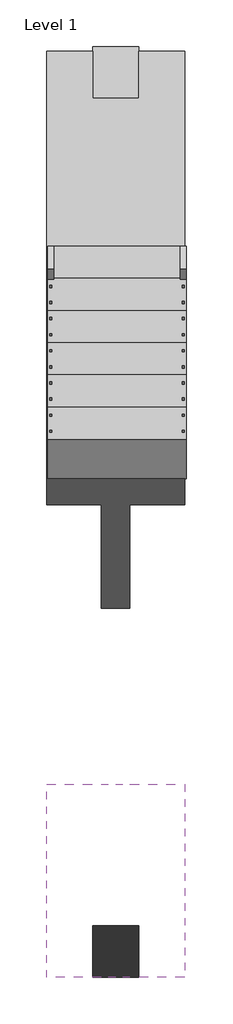
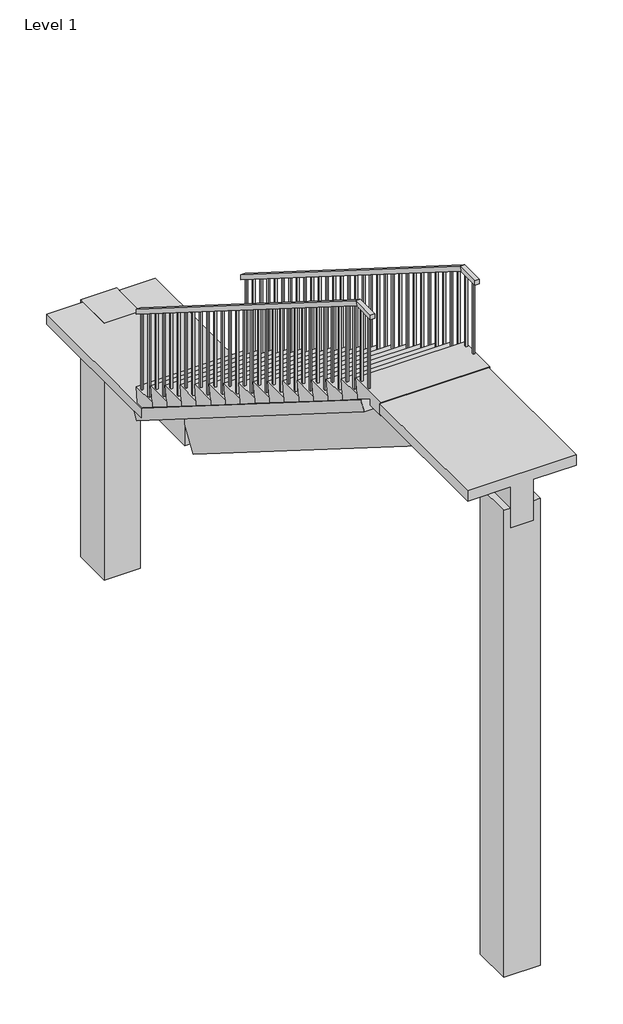
# One storey: 3 beams, 2 columns, 2 railings, 1 stair flight.
"""IFC4 building model written with IfcOpenShell, lengths in millimetres."""

from ifc_helpers import new_model, si_unit, frame, origin, place, context, project, spatial, polyline, outline, extrude, faceted_brep, element, save

model = new_model("IFC4")

# Units and contexts
model_context = context("Model", 3, world=origin())
ifc_project = project(units=[si_unit("LENGTHUNIT", "METRE", prefix="MILLI")], contexts=[model_context])

# Site, building, storey
site = spatial("IfcSite", under=ifc_project)
building = spatial("IfcBuilding", under=site)
storey = spatial("IfcBuildingStorey", under=building, Name="Level 1", Elevation=0.0)

# Beams
placement = place(None, origin())
element("IfcBeam", 1, ObjectType="Concrete-TRectangular Beam : b= 1200 x bw= 250 x tw= 120 x h=600 2", at=placement, inside=storey, context=model_context, shape_type="Brep", body=[
    faceted_brep([(2146.615308, 1121.0694774, 2541.613649), (2621.615308, 1121.0694774, 2541.613649), (2621.615308, 865.187293, 2135.5049102), (2871.615308, 865.187293, 2135.5049102), (2871.615308, 1121.0694774, 2541.613649), (3346.615308, 1121.0694774, 2541.613649), (3346.615308, 1185.0400235, 2643.1408337), (2146.615308, 1185.0400235, 2643.1408337), (3346.615308, 5379.9494631, 0.0), (2146.615308, 5379.9494631, 0.0), (3346.615308, 5468.6287248, -197.7092229), (3346.615308, 5517.5919797, -120.0), (3346.615308, 5373.0854091, -120.0), (3346.615308, 5373.0854091, 0.0), (2871.615308, 5373.0854091, -137.5090106), (2871.615308, 5468.6287248, -197.7092229), (2871.615308, 5212.7465404, -603.8179618), (2871.615308, 5373.0854091, -349.3453188), (2621.615308, 5212.7465404, -603.8179618), (2621.615308, 5373.0854091, -137.5090106), (2621.615308, 5373.0854091, -349.3453188), (2146.615308, 5468.6287248, -197.7092229), (2621.615308, 5468.6287248, -197.7092229), (2146.615308, 5373.0854091, 0.0), (2146.615308, 5373.0854091, -120.0), (2146.615308, 5517.5919797, -120.0), (2621.615308, 5517.5919797, -120.0), (2871.615308, 5373.0854091, -120.0), (2871.615308, 5517.5919797, -120.0), (2621.615308, 5373.0854091, -120.0)], [[[0, 1, 2, 3, 4, 5, 6, 7]], [[7, 6, 8, 9]], [[6, 5, 10, 11, 12, 13, 8]], [[5, 4, 14, 15, 10]], [[4, 3, 16, 17, 14]], [[3, 2, 18, 16]], [[2, 1, 19, 20, 18]], [[1, 0, 21, 22, 19]], [[0, 7, 9, 23, 24, 25, 21]], [[22, 21, 25, 26]], [[13, 23, 9, 8]], [[27, 12, 11, 28]], [[14, 27, 28, 15]], [[29, 19, 22, 26]], [[24, 29, 26, 25]], [[23, 13, 12, 27, 14, 17, 20, 19, 29, 24]], [[16, 18, 20, 17]], [[10, 15, 28, 11]]]),
])
element("IfcBeam", 2, ObjectType="Concrete-TRectangular Beam : b= 1200 x bw= 250 x tw= 120 x h=600 2", at=placement, inside=storey, context=model_context, shape_type="Brep", body=[
    faceted_brep([(2146.615308, 7193.0854091, 0.0), (2146.615308, 5379.9494631, 0.0), (2146.615308, 5373.0854091, 0.0), (3346.615308, 5373.0854091, 0.0), (3346.615308, 5379.9494631, 0.0), (3346.615308, 7193.0854091, 0.0), (2946.615308, 7193.0854091, 0.0), (2946.615308, 6785.5854091, 0.0), (2546.615308, 6785.5854091, 0.0), (2546.615308, 7193.0854091, 0.0), (3346.615308, 5373.0854091, -120.0), (3346.615308, 5517.5919797, -120.0), (3346.615308, 7193.0854091, -120.0), (2871.615308, 5373.0854091, -120.0), (2871.615308, 5517.5919797, -120.0), (2871.615308, 6785.5854091, -120.0), (2946.615308, 6785.5854091, -120.0), (2946.615308, 7193.0854091, -120.0), (2871.615308, 5373.0854091, -137.5090106), (2871.615308, 5373.0854091, -349.3453188), (2871.615308, 5373.0854091, -600.0), (2871.615308, 6785.5854091, -600.0), (2621.615308, 5373.0854091, -600.0), (2621.615308, 6785.5854091, -600.0), (2621.615308, 5373.0854091, -349.3453188), (2621.615308, 5373.0854091, -137.5090106), (2621.615308, 5373.0854091, -120.0), (2621.615308, 5517.5919797, -120.0), (2621.615308, 6785.5854091, -120.0), (2146.615308, 5373.0854091, -120.0), (2146.615308, 5517.5919797, -120.0), (2146.615308, 7193.0854091, -120.0), (2546.615308, 7193.0854091, -120.0), (2546.615308, 6785.5854091, -120.0)], [[[0, 1, 2, 3, 4, 5, 6, 7, 8, 9]], [[5, 4, 3, 10, 11, 12]], [[12, 11, 10, 13, 14, 15, 16, 17]], [[13, 18, 19, 20, 21, 15, 14]], [[20, 22, 23, 21]], [[22, 24, 25, 26, 27, 28, 23]], [[29, 30, 31, 32, 33, 28, 27, 26]], [[2, 1, 0, 31, 30, 29]], [[8, 33, 32, 9]], [[33, 8, 7, 16, 15, 21, 23, 28]], [[16, 7, 6, 17]], [[5, 12, 17, 6]], [[31, 0, 9, 32]], [[2, 29, 26, 25, 24, 22, 20, 19, 18, 13, 10, 3]]]),
])
element("IfcBeam", 3, ObjectType="Concrete-TRectangular Beam : b= 1200 x bw= 250 x tw= 120 x h=600 2", at=placement, inside=storey, context=model_context, shape_type="Brep", body=[
    faceted_brep([(2146.615308, 820.5297021, 2820.0), (3346.615308, 820.5297021, 2820.0), (3346.615308, 820.5297021, 2700.0), (2871.615308, 820.5297021, 2700.0), (2871.615308, 820.5297021, 2220.0), (2621.615308, 820.5297021, 2220.0), (2621.615308, 820.5297021, 2700.0), (2146.615308, 820.5297021, 2700.0), (2146.615308, -859.4702979, 2700.0), (2621.615308, -859.4702979, 2700.0), (2621.615308, -859.4702979, 2220.0), (2871.615308, -859.4702979, 2220.0), (2871.615308, -859.4702979, 2700.0), (3346.615308, -859.4702979, 2700.0), (3346.615308, -859.4702979, 2820.0), (2146.615308, -859.4702979, 2820.0), (2871.615308, -858.2666758, 2220.0), (2871.615308, -858.2666758, 2450.0), (2871.615308, -408.2666758, 2450.0), (2871.615308, -408.2666758, 2220.0), (2621.615308, -408.2666758, 2220.0), (2621.615308, -408.2666758, 2450.0), (2621.615308, -858.2666758, 2450.0), (2621.615308, -858.2666758, 2220.0)], [[[0, 1, 2, 3, 4, 5, 6, 7]], [[8, 9, 10, 11, 12, 13, 14, 15]], [[1, 0, 15, 14]], [[2, 1, 14, 13]], [[3, 2, 13, 12]], [[4, 3, 12, 11, 16, 17, 18, 19]], [[5, 4, 19, 20]], [[6, 5, 20, 21, 22, 23, 10, 9]], [[7, 6, 9, 8]], [[0, 7, 8, 15]], [[17, 22, 21, 18]], [[18, 21, 20, 19]], [[22, 17, 16, 23]], [[11, 10, 23, 16]]]),
])

# Columns
element("IfcColumn", 4, ObjectType="Concrete-Rectangular-Column : 400 x 450mm 2", at=placement, inside=storey, context=model_context, shape_type="Brep", body=[
    faceted_brep([(2946.615308, 7235.5854091, 0.0), (2546.615308, 7235.5854091, 0.0), (2546.615308, 7193.0854091, 0.0), (2546.615308, 6785.5854091, 0.0), (2946.615308, 6785.5854091, 0.0), (2946.615308, 7193.0854091, 0.0), (2946.615308, 7235.5854091, -3000.0), (2946.615308, 6785.5854091, -3000.0), (2546.615308, 6785.5854091, -3000.0), (2546.615308, 7235.5854091, -3000.0), (2546.615308, 6785.5854091, -120.0), (2946.615308, 6785.5854091, -120.0)], [[[0, 1, 2, 3, 4, 5]], [[6, 7, 8, 9]], [[1, 0, 6, 9]], [[3, 2, 1, 9, 8, 10]], [[4, 3, 10, 8, 7, 11]], [[0, 5, 4, 11, 7, 6]]]),
])
element("IfcColumn", 5, ObjectType="Concrete-Rectangular-Column : 400 x 450mm 2", at=placement, inside=storey, context=model_context, shape_type="Brep", body=[
    faceted_brep([(2946.615308, -408.2666758, 2450.0), (2871.615308, -408.2666758, 2450.0), (2621.615308, -408.2666758, 2450.0), (2546.615308, -408.2666758, 2450.0), (2546.615308, -858.2666758, 2450.0), (2621.615308, -858.2666758, 2450.0), (2871.615308, -858.2666758, 2450.0), (2946.615308, -858.2666758, 2450.0), (2946.615308, -408.2666758, -3000.0), (2946.615308, -858.2666758, -3000.0), (2546.615308, -858.2666758, -3000.0), (2546.615308, -408.2666758, -3000.0)], [[[0, 1, 2, 3, 4, 5, 6, 7]], [[8, 9, 10, 11]], [[3, 2, 1, 0, 8, 11]], [[4, 3, 11, 10]], [[7, 6, 5, 4, 10, 9]], [[0, 7, 9, 8]]]),
])

# Railings
element("IfcRailing", 6, ObjectType="900mm", at=placement, inside=storey, context=model_context, shape_type="SolidModel", body=[
    faceted_brep([(2208.2375205, 5500.0919589, 1076.4705882), (2208.2375205, 5500.0919589, 1017.3686062), (2158.2375205, 5500.0919589, 1017.3686062), (2158.2375205, 5500.0919589, 1076.4705882), (2208.2375205, 1300.0919589, 3723.5294118), (2208.2375205, 1285.6501475, 3673.5294118), (2158.2375205, 1285.6501475, 3673.5294118), (2158.2375205, 1300.0919589, 3723.5294118), (2208.2375205, 1020.0919589, 3723.5294118), (2158.2375205, 1020.0919589, 3723.5294118), (2158.2375205, 1020.0919589, 3673.5294118), (2208.2375205, 1020.0919589, 3673.5294118)], [[[0, 1, 2, 3]], [[1, 0, 4, 5]], [[2, 1, 5, 6]], [[3, 2, 6, 7]], [[0, 3, 7, 4]], [[8, 9, 10, 11]], [[5, 4, 8, 11]], [[6, 5, 11, 10]], [[7, 6, 10, 9]], [[4, 7, 9, 8]]]),
    extrude(outline(polyline([(2173.2375205, 1100.0919589), (2193.2375205, 1100.0919589), (2193.2375205, 1080.0919589), (2173.2375205, 1080.0919589), (2173.2375205, 1100.0919589)])), frame((0.0, 0.0, 2823.5294118), z_axis=(0.0, 0.0, 1.0), x_axis=(1.0, 0.0, 0.0)), (0.0, 0.0, 1.0), 850.0),
    extrude(outline(polyline([(2173.2375205, 1240.0919589), (2193.2375205, 1240.0919589), (2193.2375205, 1220.0919589), (2173.2375205, 1220.0919589), (2173.2375205, 1240.0919589)])), frame((0.0, 0.0, 2823.5294118), z_axis=(0.0, 0.0, 1.0), x_axis=(1.0, 0.0, 0.0)), (0.0, 0.0, 1.0), 850.0),
    extrude(outline(polyline([(1380.0919589, 3614.0072617), (1380.0919589, 2647.0588235), (1360.0919589, 2647.0588235), (1360.0919589, 3626.6123037), (1380.0919589, 3614.0072617)])), frame((2173.2375205, 0.0, 0.0), z_axis=(1.0, 0.0, 0.0), x_axis=(0.0, 1.0, 0.0)), (0.0, 0.0, 1.0), 20.0),
    extrude(outline(polyline([(1520.0919589, 3525.7719676), (1520.0919589, 2647.0588235), (1500.0919589, 2647.0588235), (1500.0919589, 3538.3770096), (1520.0919589, 3525.7719676)])), frame((2173.2375205, 0.0, 0.0), z_axis=(1.0, 0.0, 0.0), x_axis=(0.0, 1.0, 0.0)), (0.0, 0.0, 1.0), 20.0),
    extrude(outline(polyline([(1660.0919589, 3437.5366735), (1660.0919589, 2470.5882353), (1640.0919589, 2470.5882353), (1640.0919589, 3450.1417155), (1660.0919589, 3437.5366735)])), frame((2173.2375205, 0.0, 0.0), z_axis=(1.0, 0.0, 0.0), x_axis=(0.0, 1.0, 0.0)), (0.0, 0.0, 1.0), 20.0),
    extrude(outline(polyline([(1800.0919589, 3349.3013793), (1800.0919589, 2470.5882353), (1780.0919589, 2470.5882353), (1780.0919589, 3361.9064214), (1800.0919589, 3349.3013793)])), frame((2173.2375205, 0.0, 0.0), z_axis=(1.0, 0.0, 0.0), x_axis=(0.0, 1.0, 0.0)), (0.0, 0.0, 1.0), 20.0),
    extrude(outline(polyline([(1940.0919589, 3261.0660852), (1940.0919589, 2294.1176471), (1920.0919589, 2294.1176471), (1920.0919589, 3273.6711272), (1940.0919589, 3261.0660852)])), frame((2173.2375205, 0.0, 0.0), z_axis=(1.0, 0.0, 0.0), x_axis=(0.0, 1.0, 0.0)), (0.0, 0.0, 1.0), 20.0),
    extrude(outline(polyline([(2080.0919589, 3172.8307911), (2080.0919589, 2294.1176471), (2060.0919589, 2294.1176471), (2060.0919589, 3185.4358331), (2080.0919589, 3172.8307911)])), frame((2173.2375205, 0.0, 0.0), z_axis=(1.0, 0.0, 0.0), x_axis=(0.0, 1.0, 0.0)), (0.0, 0.0, 1.0), 20.0),
    extrude(outline(polyline([(2220.0919589, 3084.595497), (2220.0919589, 2117.6470588), (2200.0919589, 2117.6470588), (2200.0919589, 3097.200539), (2220.0919589, 3084.595497)])), frame((2173.2375205, 0.0, 0.0), z_axis=(1.0, 0.0, 0.0), x_axis=(0.0, 1.0, 0.0)), (0.0, 0.0, 1.0), 20.0),
    extrude(outline(polyline([(2360.0919589, 2996.3602029), (2360.0919589, 2117.6470588), (2340.0919589, 2117.6470588), (2340.0919589, 3008.9652449), (2360.0919589, 2996.3602029)])), frame((2173.2375205, 0.0, 0.0), z_axis=(1.0, 0.0, 0.0), x_axis=(0.0, 1.0, 0.0)), (0.0, 0.0, 1.0), 20.0),
    extrude(outline(polyline([(2500.0919589, 2908.1249088), (2500.0919589, 1941.1764706), (2480.0919589, 1941.1764706), (2480.0919589, 2920.7299508), (2500.0919589, 2908.1249088)])), frame((2173.2375205, 0.0, 0.0), z_axis=(1.0, 0.0, 0.0), x_axis=(0.0, 1.0, 0.0)), (0.0, 0.0, 1.0), 20.0),
    extrude(outline(polyline([(2640.0919589, 2819.8896146), (2640.0919589, 1941.1764706), (2620.0919589, 1941.1764706), (2620.0919589, 2832.4946567), (2640.0919589, 2819.8896146)])), frame((2173.2375205, 0.0, 0.0), z_axis=(1.0, 0.0, 0.0), x_axis=(0.0, 1.0, 0.0)), (0.0, 0.0, 1.0), 20.0),
    extrude(outline(polyline([(2780.0919589, 2731.6543205), (2780.0919589, 1764.7058824), (2760.0919589, 1764.7058824), (2760.0919589, 2744.2593625), (2780.0919589, 2731.6543205)])), frame((2173.2375205, 0.0, 0.0), z_axis=(1.0, 0.0, 0.0), x_axis=(0.0, 1.0, 0.0)), (0.0, 0.0, 1.0), 20.0),
    extrude(outline(polyline([(2920.0919589, 2643.4190264), (2920.0919589, 1764.7058824), (2900.0919589, 1764.7058824), (2900.0919589, 2656.0240684), (2920.0919589, 2643.4190264)])), frame((2173.2375205, 0.0, 0.0), z_axis=(1.0, 0.0, 0.0), x_axis=(0.0, 1.0, 0.0)), (0.0, 0.0, 1.0), 20.0),
    extrude(outline(polyline([(3060.0919589, 2555.1837323), (3060.0919589, 1588.2352941), (3040.0919589, 1588.2352941), (3040.0919589, 2567.7887743), (3060.0919589, 2555.1837323)])), frame((2173.2375205, 0.0, 0.0), z_axis=(1.0, 0.0, 0.0), x_axis=(0.0, 1.0, 0.0)), (0.0, 0.0, 1.0), 20.0),
    extrude(outline(polyline([(3200.0919589, 2466.9484382), (3200.0919589, 1588.2352941), (3180.0919589, 1588.2352941), (3180.0919589, 2479.5534802), (3200.0919589, 2466.9484382)])), frame((2173.2375205, 0.0, 0.0), z_axis=(1.0, 0.0, 0.0), x_axis=(0.0, 1.0, 0.0)), (0.0, 0.0, 1.0), 20.0),
    extrude(outline(polyline([(3340.0919589, 2378.713144), (3340.0919589, 1411.7647059), (3320.0919589, 1411.7647059), (3320.0919589, 2391.3181861), (3340.0919589, 2378.713144)])), frame((2173.2375205, 0.0, 0.0), z_axis=(1.0, 0.0, 0.0), x_axis=(0.0, 1.0, 0.0)), (0.0, 0.0, 1.0), 20.0),
    extrude(outline(polyline([(3480.0919589, 2290.4778499), (3480.0919589, 1411.7647059), (3460.0919589, 1411.7647059), (3460.0919589, 2303.0828919), (3480.0919589, 2290.4778499)])), frame((2173.2375205, 0.0, 0.0), z_axis=(1.0, 0.0, 0.0), x_axis=(0.0, 1.0, 0.0)), (0.0, 0.0, 1.0), 20.0),
    extrude(outline(polyline([(3620.0919589, 2202.2425558), (3620.0919589, 1235.2941176), (3600.0919589, 1235.2941176), (3600.0919589, 2214.8475978), (3620.0919589, 2202.2425558)])), frame((2173.2375205, 0.0, 0.0), z_axis=(1.0, 0.0, 0.0), x_axis=(0.0, 1.0, 0.0)), (0.0, 0.0, 1.0), 20.0),
    extrude(outline(polyline([(3760.0919589, 2114.0072617), (3760.0919589, 1235.2941176), (3740.0919589, 1235.2941176), (3740.0919589, 2126.6123037), (3760.0919589, 2114.0072617)])), frame((2173.2375205, 0.0, 0.0), z_axis=(1.0, 0.0, 0.0), x_axis=(0.0, 1.0, 0.0)), (0.0, 0.0, 1.0), 20.0),
    extrude(outline(polyline([(3900.0919589, 2025.7719676), (3900.0919589, 1058.8235294), (3880.0919589, 1058.8235294), (3880.0919589, 2038.3770096), (3900.0919589, 2025.7719676)])), frame((2173.2375205, 0.0, 0.0), z_axis=(1.0, 0.0, 0.0), x_axis=(0.0, 1.0, 0.0)), (0.0, 0.0, 1.0), 20.0),
    extrude(outline(polyline([(4040.0919589, 1937.5366735), (4040.0919589, 1058.8235294), (4020.0919589, 1058.8235294), (4020.0919589, 1950.1417155), (4040.0919589, 1937.5366735)])), frame((2173.2375205, 0.0, 0.0), z_axis=(1.0, 0.0, 0.0), x_axis=(0.0, 1.0, 0.0)), (0.0, 0.0, 1.0), 20.0),
    extrude(outline(polyline([(4180.0919589, 1849.3013793), (4180.0919589, 882.3529412), (4160.0919589, 882.3529412), (4160.0919589, 1861.9064214), (4180.0919589, 1849.3013793)])), frame((2173.2375205, 0.0, 0.0), z_axis=(1.0, 0.0, 0.0), x_axis=(0.0, 1.0, 0.0)), (0.0, 0.0, 1.0), 20.0),
    extrude(outline(polyline([(4320.0919589, 1761.0660852), (4320.0919589, 882.3529412), (4300.0919589, 882.3529412), (4300.0919589, 1773.6711272), (4320.0919589, 1761.0660852)])), frame((2173.2375205, 0.0, 0.0), z_axis=(1.0, 0.0, 0.0), x_axis=(0.0, 1.0, 0.0)), (0.0, 0.0, 1.0), 20.0),
    extrude(outline(polyline([(4460.0919589, 1672.8307911), (4460.0919589, 705.8823529), (4440.0919589, 705.8823529), (4440.0919589, 1685.4358331), (4460.0919589, 1672.8307911)])), frame((2173.2375205, 0.0, 0.0), z_axis=(1.0, 0.0, 0.0), x_axis=(0.0, 1.0, 0.0)), (0.0, 0.0, 1.0), 20.0),
    extrude(outline(polyline([(4600.0919589, 1584.595497), (4600.0919589, 705.8823529), (4580.0919589, 705.8823529), (4580.0919589, 1597.200539), (4600.0919589, 1584.595497)])), frame((2173.2375205, 0.0, 0.0), z_axis=(1.0, 0.0, 0.0), x_axis=(0.0, 1.0, 0.0)), (0.0, 0.0, 1.0), 20.0),
    extrude(outline(polyline([(4740.0919589, 1496.3602029), (4740.0919589, 529.4117647), (4720.0919589, 529.4117647), (4720.0919589, 1508.9652449), (4740.0919589, 1496.3602029)])), frame((2173.2375205, 0.0, 0.0), z_axis=(1.0, 0.0, 0.0), x_axis=(0.0, 1.0, 0.0)), (0.0, 0.0, 1.0), 20.0),
    extrude(outline(polyline([(4880.0919589, 1408.1249088), (4880.0919589, 529.4117647), (4860.0919589, 529.4117647), (4860.0919589, 1420.7299508), (4880.0919589, 1408.1249088)])), frame((2173.2375205, 0.0, 0.0), z_axis=(1.0, 0.0, 0.0), x_axis=(0.0, 1.0, 0.0)), (0.0, 0.0, 1.0), 20.0),
    extrude(outline(polyline([(5020.0919589, 1319.8896146), (5020.0919589, 352.9411765), (5000.0919589, 352.9411765), (5000.0919589, 1332.4946567), (5020.0919589, 1319.8896146)])), frame((2173.2375205, 0.0, 0.0), z_axis=(1.0, 0.0, 0.0), x_axis=(0.0, 1.0, 0.0)), (0.0, 0.0, 1.0), 20.0),
    extrude(outline(polyline([(5160.0919589, 1231.6543205), (5160.0919589, 352.9411765), (5140.0919589, 352.9411765), (5140.0919589, 1244.2593625), (5160.0919589, 1231.6543205)])), frame((2173.2375205, 0.0, 0.0), z_axis=(1.0, 0.0, 0.0), x_axis=(0.0, 1.0, 0.0)), (0.0, 0.0, 1.0), 20.0),
    extrude(outline(polyline([(5300.0919589, 1143.4190264), (5300.0919589, 176.4705882), (5280.0919589, 176.4705882), (5280.0919589, 1156.0240684), (5300.0919589, 1143.4190264)])), frame((2173.2375205, 0.0, 0.0), z_axis=(1.0, 0.0, 0.0), x_axis=(0.0, 1.0, 0.0)), (0.0, 0.0, 1.0), 20.0),
    extrude(outline(polyline([(5440.0919589, 1055.1837323), (5440.0919589, 176.4705882), (5420.0919589, 176.4705882), (5420.0919589, 1067.7887743), (5440.0919589, 1055.1837323)])), frame((2173.2375205, 0.0, 0.0), z_axis=(1.0, 0.0, 0.0), x_axis=(0.0, 1.0, 0.0)), (0.0, 0.0, 1.0), 20.0),
])
element("IfcRailing", 7, ObjectType="900mm", at=placement, inside=storey, context=model_context, shape_type="SolidModel", body=[
    faceted_brep([(3360.4586748, 5500.0919589, 1076.4705882), (3360.4586748, 5500.0919589, 1017.3686062), (3310.4586748, 5500.0919589, 1017.3686062), (3310.4586748, 5500.0919589, 1076.4705882), (3360.4586748, 1300.0919589, 3723.5294118), (3360.4586748, 1285.6501475, 3673.5294118), (3310.4586748, 1285.6501475, 3673.5294118), (3310.4586748, 1300.0919589, 3723.5294118), (3360.4586748, 1020.0919589, 3723.5294118), (3310.4586748, 1020.0919589, 3723.5294118), (3310.4586748, 1020.0919589, 3673.5294118), (3360.4586748, 1020.0919589, 3673.5294118)], [[[0, 1, 2, 3]], [[1, 0, 4, 5]], [[2, 1, 5, 6]], [[3, 2, 6, 7]], [[0, 3, 7, 4]], [[8, 9, 10, 11]], [[5, 4, 8, 11]], [[6, 5, 11, 10]], [[7, 6, 10, 9]], [[4, 7, 9, 8]]]),
    extrude(outline(polyline([(3345.4586748, 1100.0919589), (3345.4586748, 1080.0919589), (3325.4586748, 1080.0919589), (3325.4586748, 1100.0919589), (3345.4586748, 1100.0919589)])), frame((0.0, 0.0, 2823.5294118), z_axis=(0.0, 0.0, 1.0), x_axis=(1.0, 0.0, 0.0)), (0.0, 0.0, 1.0), 850.0),
    extrude(outline(polyline([(3345.4586748, 1240.0919589), (3345.4586748, 1220.0919589), (3325.4586748, 1220.0919589), (3325.4586748, 1240.0919589), (3345.4586748, 1240.0919589)])), frame((0.0, 0.0, 2823.5294118), z_axis=(0.0, 0.0, 1.0), x_axis=(1.0, 0.0, 0.0)), (0.0, 0.0, 1.0), 850.0),
    extrude(outline(polyline([(1380.0919589, 2647.0588235), (1360.0919589, 2647.0588235), (1360.0919589, 3626.6123037), (1380.0919589, 3614.0072617), (1380.0919589, 2647.0588235)])), frame((3325.4586748, 0.0, 0.0), z_axis=(1.0, 0.0, 0.0), x_axis=(0.0, 1.0, 0.0)), (0.0, 0.0, 1.0), 20.0),
    extrude(outline(polyline([(1520.0919589, 2647.0588235), (1500.0919589, 2647.0588235), (1500.0919589, 3538.3770096), (1520.0919589, 3525.7719676), (1520.0919589, 2647.0588235)])), frame((3325.4586748, 0.0, 0.0), z_axis=(1.0, 0.0, 0.0), x_axis=(0.0, 1.0, 0.0)), (0.0, 0.0, 1.0), 20.0),
    extrude(outline(polyline([(1660.0919589, 2470.5882353), (1640.0919589, 2470.5882353), (1640.0919589, 3450.1417155), (1660.0919589, 3437.5366735), (1660.0919589, 2470.5882353)])), frame((3325.4586748, 0.0, 0.0), z_axis=(1.0, 0.0, 0.0), x_axis=(0.0, 1.0, 0.0)), (0.0, 0.0, 1.0), 20.0),
    extrude(outline(polyline([(1800.0919589, 2470.5882353), (1780.0919589, 2470.5882353), (1780.0919589, 3361.9064214), (1800.0919589, 3349.3013793), (1800.0919589, 2470.5882353)])), frame((3325.4586748, 0.0, 0.0), z_axis=(1.0, 0.0, 0.0), x_axis=(0.0, 1.0, 0.0)), (0.0, 0.0, 1.0), 20.0),
    extrude(outline(polyline([(1940.0919589, 2294.1176471), (1920.0919589, 2294.1176471), (1920.0919589, 3273.6711272), (1940.0919589, 3261.0660852), (1940.0919589, 2294.1176471)])), frame((3325.4586748, 0.0, 0.0), z_axis=(1.0, 0.0, 0.0), x_axis=(0.0, 1.0, 0.0)), (0.0, 0.0, 1.0), 20.0),
    extrude(outline(polyline([(2080.0919589, 2294.1176471), (2060.0919589, 2294.1176471), (2060.0919589, 3185.4358331), (2080.0919589, 3172.8307911), (2080.0919589, 2294.1176471)])), frame((3325.4586748, 0.0, 0.0), z_axis=(1.0, 0.0, 0.0), x_axis=(0.0, 1.0, 0.0)), (0.0, 0.0, 1.0), 20.0),
    extrude(outline(polyline([(2220.0919589, 2117.6470588), (2200.0919589, 2117.6470588), (2200.0919589, 3097.200539), (2220.0919589, 3084.595497), (2220.0919589, 2117.6470588)])), frame((3325.4586748, 0.0, 0.0), z_axis=(1.0, 0.0, 0.0), x_axis=(0.0, 1.0, 0.0)), (0.0, 0.0, 1.0), 20.0),
    extrude(outline(polyline([(2360.0919589, 2117.6470588), (2340.0919589, 2117.6470588), (2340.0919589, 3008.9652449), (2360.0919589, 2996.3602029), (2360.0919589, 2117.6470588)])), frame((3325.4586748, 0.0, 0.0), z_axis=(1.0, 0.0, 0.0), x_axis=(0.0, 1.0, 0.0)), (0.0, 0.0, 1.0), 20.0),
    extrude(outline(polyline([(2500.0919589, 1941.1764706), (2480.0919589, 1941.1764706), (2480.0919589, 2920.7299508), (2500.0919589, 2908.1249088), (2500.0919589, 1941.1764706)])), frame((3325.4586748, 0.0, 0.0), z_axis=(1.0, 0.0, 0.0), x_axis=(0.0, 1.0, 0.0)), (0.0, 0.0, 1.0), 20.0),
    extrude(outline(polyline([(2640.0919589, 1941.1764706), (2620.0919589, 1941.1764706), (2620.0919589, 2832.4946567), (2640.0919589, 2819.8896146), (2640.0919589, 1941.1764706)])), frame((3325.4586748, 0.0, 0.0), z_axis=(1.0, 0.0, 0.0), x_axis=(0.0, 1.0, 0.0)), (0.0, 0.0, 1.0), 20.0),
    extrude(outline(polyline([(2780.0919589, 1764.7058824), (2760.0919589, 1764.7058824), (2760.0919589, 2744.2593625), (2780.0919589, 2731.6543205), (2780.0919589, 1764.7058824)])), frame((3325.4586748, 0.0, 0.0), z_axis=(1.0, 0.0, 0.0), x_axis=(0.0, 1.0, 0.0)), (0.0, 0.0, 1.0), 20.0),
    extrude(outline(polyline([(2920.0919589, 1764.7058824), (2900.0919589, 1764.7058824), (2900.0919589, 2656.0240684), (2920.0919589, 2643.4190264), (2920.0919589, 1764.7058824)])), frame((3325.4586748, 0.0, 0.0), z_axis=(1.0, 0.0, 0.0), x_axis=(0.0, 1.0, 0.0)), (0.0, 0.0, 1.0), 20.0),
    extrude(outline(polyline([(3060.0919589, 1588.2352941), (3040.0919589, 1588.2352941), (3040.0919589, 2567.7887743), (3060.0919589, 2555.1837323), (3060.0919589, 1588.2352941)])), frame((3325.4586748, 0.0, 0.0), z_axis=(1.0, 0.0, 0.0), x_axis=(0.0, 1.0, 0.0)), (0.0, 0.0, 1.0), 20.0),
    extrude(outline(polyline([(3200.0919589, 1588.2352941), (3180.0919589, 1588.2352941), (3180.0919589, 2479.5534802), (3200.0919589, 2466.9484382), (3200.0919589, 1588.2352941)])), frame((3325.4586748, 0.0, 0.0), z_axis=(1.0, 0.0, 0.0), x_axis=(0.0, 1.0, 0.0)), (0.0, 0.0, 1.0), 20.0),
    extrude(outline(polyline([(3340.0919589, 1411.7647059), (3320.0919589, 1411.7647059), (3320.0919589, 2391.3181861), (3340.0919589, 2378.713144), (3340.0919589, 1411.7647059)])), frame((3325.4586748, 0.0, 0.0), z_axis=(1.0, 0.0, 0.0), x_axis=(0.0, 1.0, 0.0)), (0.0, 0.0, 1.0), 20.0),
    extrude(outline(polyline([(3480.0919589, 1411.7647059), (3460.0919589, 1411.7647059), (3460.0919589, 2303.0828919), (3480.0919589, 2290.4778499), (3480.0919589, 1411.7647059)])), frame((3325.4586748, 0.0, 0.0), z_axis=(1.0, 0.0, 0.0), x_axis=(0.0, 1.0, 0.0)), (0.0, 0.0, 1.0), 20.0),
    extrude(outline(polyline([(3620.0919589, 1235.2941176), (3600.0919589, 1235.2941176), (3600.0919589, 2214.8475978), (3620.0919589, 2202.2425558), (3620.0919589, 1235.2941176)])), frame((3325.4586748, 0.0, 0.0), z_axis=(1.0, 0.0, 0.0), x_axis=(0.0, 1.0, 0.0)), (0.0, 0.0, 1.0), 20.0),
    extrude(outline(polyline([(3760.0919589, 1235.2941176), (3740.0919589, 1235.2941176), (3740.0919589, 2126.6123037), (3760.0919589, 2114.0072617), (3760.0919589, 1235.2941176)])), frame((3325.4586748, 0.0, 0.0), z_axis=(1.0, 0.0, 0.0), x_axis=(0.0, 1.0, 0.0)), (0.0, 0.0, 1.0), 20.0),
    extrude(outline(polyline([(3900.0919589, 1058.8235294), (3880.0919589, 1058.8235294), (3880.0919589, 2038.3770096), (3900.0919589, 2025.7719676), (3900.0919589, 1058.8235294)])), frame((3325.4586748, 0.0, 0.0), z_axis=(1.0, 0.0, 0.0), x_axis=(0.0, 1.0, 0.0)), (0.0, 0.0, 1.0), 20.0),
    extrude(outline(polyline([(4040.0919589, 1058.8235294), (4020.0919589, 1058.8235294), (4020.0919589, 1950.1417155), (4040.0919589, 1937.5366735), (4040.0919589, 1058.8235294)])), frame((3325.4586748, 0.0, 0.0), z_axis=(1.0, 0.0, 0.0), x_axis=(0.0, 1.0, 0.0)), (0.0, 0.0, 1.0), 20.0),
    extrude(outline(polyline([(4180.0919589, 882.3529412), (4160.0919589, 882.3529412), (4160.0919589, 1861.9064214), (4180.0919589, 1849.3013793), (4180.0919589, 882.3529412)])), frame((3325.4586748, 0.0, 0.0), z_axis=(1.0, 0.0, 0.0), x_axis=(0.0, 1.0, 0.0)), (0.0, 0.0, 1.0), 20.0),
    extrude(outline(polyline([(4320.0919589, 882.3529412), (4300.0919589, 882.3529412), (4300.0919589, 1773.6711272), (4320.0919589, 1761.0660852), (4320.0919589, 882.3529412)])), frame((3325.4586748, 0.0, 0.0), z_axis=(1.0, 0.0, 0.0), x_axis=(0.0, 1.0, 0.0)), (0.0, 0.0, 1.0), 20.0),
    extrude(outline(polyline([(4460.0919589, 705.8823529), (4440.0919589, 705.8823529), (4440.0919589, 1685.4358331), (4460.0919589, 1672.8307911), (4460.0919589, 705.8823529)])), frame((3325.4586748, 0.0, 0.0), z_axis=(1.0, 0.0, 0.0), x_axis=(0.0, 1.0, 0.0)), (0.0, 0.0, 1.0), 20.0),
    extrude(outline(polyline([(4600.0919589, 705.8823529), (4580.0919589, 705.8823529), (4580.0919589, 1597.200539), (4600.0919589, 1584.595497), (4600.0919589, 705.8823529)])), frame((3325.4586748, 0.0, 0.0), z_axis=(1.0, 0.0, 0.0), x_axis=(0.0, 1.0, 0.0)), (0.0, 0.0, 1.0), 20.0),
    extrude(outline(polyline([(4740.0919589, 529.4117647), (4720.0919589, 529.4117647), (4720.0919589, 1508.9652449), (4740.0919589, 1496.3602029), (4740.0919589, 529.4117647)])), frame((3325.4586748, 0.0, 0.0), z_axis=(1.0, 0.0, 0.0), x_axis=(0.0, 1.0, 0.0)), (0.0, 0.0, 1.0), 20.0),
    extrude(outline(polyline([(4880.0919589, 529.4117647), (4860.0919589, 529.4117647), (4860.0919589, 1420.7299508), (4880.0919589, 1408.1249088), (4880.0919589, 529.4117647)])), frame((3325.4586748, 0.0, 0.0), z_axis=(1.0, 0.0, 0.0), x_axis=(0.0, 1.0, 0.0)), (0.0, 0.0, 1.0), 20.0),
    extrude(outline(polyline([(5020.0919589, 352.9411765), (5000.0919589, 352.9411765), (5000.0919589, 1332.4946567), (5020.0919589, 1319.8896146), (5020.0919589, 352.9411765)])), frame((3325.4586748, 0.0, 0.0), z_axis=(1.0, 0.0, 0.0), x_axis=(0.0, 1.0, 0.0)), (0.0, 0.0, 1.0), 20.0),
    extrude(outline(polyline([(5160.0919589, 352.9411765), (5140.0919589, 352.9411765), (5140.0919589, 1244.2593625), (5160.0919589, 1231.6543205), (5160.0919589, 352.9411765)])), frame((3325.4586748, 0.0, 0.0), z_axis=(1.0, 0.0, 0.0), x_axis=(0.0, 1.0, 0.0)), (0.0, 0.0, 1.0), 20.0),
    extrude(outline(polyline([(5300.0919589, 176.4705882), (5280.0919589, 176.4705882), (5280.0919589, 1156.0240684), (5300.0919589, 1143.4190264), (5300.0919589, 176.4705882)])), frame((3325.4586748, 0.0, 0.0), z_axis=(1.0, 0.0, 0.0), x_axis=(0.0, 1.0, 0.0)), (0.0, 0.0, 1.0), 20.0),
    extrude(outline(polyline([(5440.0919589, 176.4705882), (5420.0919589, 176.4705882), (5420.0919589, 1067.7887743), (5440.0919589, 1055.1837323), (5440.0919589, 176.4705882)])), frame((3325.4586748, 0.0, 0.0), z_axis=(1.0, 0.0, 0.0), x_axis=(0.0, 1.0, 0.0)), (0.0, 0.0, 1.0), 20.0),
])

# Stair flight
element("IfcStairFlight", 8, ObjectType="25 mm Nosing", at=placement, inside=storey, context=model_context, shape_type="Brep", body=[
    faceted_brep([(2157.8375205, 5500.0919589, 176.4705882), (3360.8586748, 5500.0919589, 176.4705882), (3360.8586748, 5475.0919589, 0.0), (2157.8375205, 5475.0919589, 0.0), (2157.8375205, 5195.0919589, 176.4705882), (3360.8586748, 5195.0919589, 176.4705882), (3360.8586748, 5195.0919589, 117.3686062), (3360.8586748, 5381.3168141, 0.0), (2157.8375205, 5381.3168141, 0.0), (2157.8375205, 5195.0919589, 117.3686062), (3360.8586748, 5220.0919589, 352.9411765), (2157.8375205, 5220.0919589, 352.9411765), (2157.8375205, 4915.0919589, 352.9411765), (3360.8586748, 4915.0919589, 352.9411765), (3360.8586748, 4915.0919589, 293.8391945), (2157.8375205, 4915.0919589, 293.8391945), (3360.8586748, 4940.0919589, 529.4117647), (2157.8375205, 4940.0919589, 529.4117647), (2157.8375205, 4635.0919589, 529.4117647), (3360.8586748, 4635.0919589, 529.4117647), (3360.8586748, 4635.0919589, 470.3097827), (2157.8375205, 4635.0919589, 470.3097827), (3360.8586748, 4660.0919589, 705.8823529), (2157.8375205, 4660.0919589, 705.8823529), (2157.8375205, 4355.0919589, 705.8823529), (3360.8586748, 4355.0919589, 705.8823529), (3360.8586748, 4355.0919589, 646.7803709), (2157.8375205, 4355.0919589, 646.7803709), (3360.8586748, 4380.0919589, 882.3529412), (2157.8375205, 4380.0919589, 882.3529412), (2157.8375205, 4075.0919589, 882.3529412), (3360.8586748, 4075.0919589, 882.3529412), (3360.8586748, 4075.0919589, 823.2509592), (2157.8375205, 4075.0919589, 823.2509592), (3360.8586748, 4100.0919589, 1058.8235294), (2157.8375205, 4100.0919589, 1058.8235294), (2157.8375205, 3795.0919589, 1058.8235294), (3360.8586748, 3795.0919589, 1058.8235294), (3360.8586748, 3795.0919589, 999.7215474), (2157.8375205, 3795.0919589, 999.7215474), (3360.8586748, 3820.0919589, 1235.2941176), (2157.8375205, 3820.0919589, 1235.2941176), (2157.8375205, 3515.0919589, 1235.2941176), (3360.8586748, 3515.0919589, 1235.2941176), (3360.8586748, 3515.0919589, 1176.1921356), (2157.8375205, 3515.0919589, 1176.1921356), (3360.8586748, 3540.0919589, 1411.7647059), (2157.8375205, 3540.0919589, 1411.7647059), (2157.8375205, 3235.0919589, 1411.7647059), (3360.8586748, 3235.0919589, 1411.7647059), (3360.8586748, 3235.0919589, 1352.6627239), (2157.8375205, 3235.0919589, 1352.6627239), (3360.8586748, 3260.0919589, 1588.2352941), (2157.8375205, 3260.0919589, 1588.2352941), (2157.8375205, 2955.0919589, 1588.2352941), (3360.8586748, 2955.0919589, 1588.2352941), (3360.8586748, 2955.0919589, 1529.1333121), (2157.8375205, 2955.0919589, 1529.1333121), (3360.8586748, 2980.0919589, 1764.7058824), (2157.8375205, 2980.0919589, 1764.7058824), (2157.8375205, 2675.0919589, 1764.7058824), (3360.8586748, 2675.0919589, 1764.7058824), (3360.8586748, 2675.0919589, 1705.6039004), (2157.8375205, 2675.0919589, 1705.6039004), (3360.8586748, 2700.0919589, 1941.1764706), (2157.8375205, 2700.0919589, 1941.1764706), (2157.8375205, 2395.0919589, 1941.1764706), (3360.8586748, 2395.0919589, 1941.1764706), (3360.8586748, 2395.0919589, 1882.0744886), (2157.8375205, 2395.0919589, 1882.0744886), (3360.8586748, 2420.0919589, 2117.6470588), (2157.8375205, 2420.0919589, 2117.6470588), (2157.8375205, 2115.0919589, 2117.6470588), (3360.8586748, 2115.0919589, 2117.6470588), (3360.8586748, 2115.0919589, 2058.5450768), (2157.8375205, 2115.0919589, 2058.5450768), (3360.8586748, 2140.0919589, 2294.1176471), (2157.8375205, 2140.0919589, 2294.1176471), (2157.8375205, 1835.0919589, 2294.1176471), (3360.8586748, 1835.0919589, 2294.1176471), (3360.8586748, 1835.0919589, 2235.0156651), (2157.8375205, 1835.0919589, 2235.0156651), (3360.8586748, 1860.0919589, 2470.5882353), (2157.8375205, 1860.0919589, 2470.5882353), (2157.8375205, 1555.0919589, 2470.5882353), (3360.8586748, 1555.0919589, 2470.5882353), (3360.8586748, 1555.0919589, 2411.4862533), (2157.8375205, 1555.0919589, 2411.4862533), (3360.8586748, 1580.0919589, 2647.0588235), (2157.8375205, 1580.0919589, 2647.0588235), (2157.8375205, 1275.0919589, 2647.0588235), (3360.8586748, 1275.0919589, 2647.0588235), (3360.8586748, 1275.0919589, 2587.9568415), (2157.8375205, 1275.0919589, 2587.9568415), (3360.8586748, 1300.0919589, 2823.5294118), (2157.8375205, 1300.0919589, 2823.5294118), (2157.8375205, 820.0919589, 2823.5294118), (3360.8586748, 820.0919589, 2823.5294118), (3360.8586748, 820.0919589, 2673.5294118), (3360.8586748, 1020.0919589, 2673.5294118), (3360.8586748, 1020.0919589, 2748.6711272), (2157.8375205, 1020.0919589, 2748.6711272), (2157.8375205, 1020.0919589, 2673.5294118), (2157.8375205, 820.0919589, 2673.5294118)], [[[0, 1, 2, 3]], [[1, 0, 4, 5]], [[1, 5, 6, 7, 2]], [[4, 0, 3, 8, 9]], [[10, 11, 12, 13]], [[10, 13, 14, 6, 5]], [[12, 11, 4, 9, 15]], [[5, 4, 11, 10]], [[16, 17, 18, 19]], [[16, 19, 20, 14, 13]], [[18, 17, 12, 15, 21]], [[13, 12, 17, 16]], [[22, 23, 24, 25]], [[22, 25, 26, 20, 19]], [[24, 23, 18, 21, 27]], [[19, 18, 23, 22]], [[28, 29, 30, 31]], [[28, 31, 32, 26, 25]], [[30, 29, 24, 27, 33]], [[25, 24, 29, 28]], [[34, 35, 36, 37]], [[34, 37, 38, 32, 31]], [[36, 35, 30, 33, 39]], [[31, 30, 35, 34]], [[40, 41, 42, 43]], [[40, 43, 44, 38, 37]], [[42, 41, 36, 39, 45]], [[37, 36, 41, 40]], [[46, 47, 48, 49]], [[46, 49, 50, 44, 43]], [[48, 47, 42, 45, 51]], [[43, 42, 47, 46]], [[52, 53, 54, 55]], [[52, 55, 56, 50, 49]], [[54, 53, 48, 51, 57]], [[49, 48, 53, 52]], [[58, 59, 60, 61]], [[58, 61, 62, 56, 55]], [[60, 59, 54, 57, 63]], [[55, 54, 59, 58]], [[64, 65, 66, 67]], [[64, 67, 68, 62, 61]], [[66, 65, 60, 63, 69]], [[61, 60, 65, 64]], [[70, 71, 72, 73]], [[70, 73, 74, 68, 67]], [[72, 71, 66, 69, 75]], [[67, 66, 71, 70]], [[76, 77, 78, 79]], [[76, 79, 80, 74, 73]], [[78, 77, 72, 75, 81]], [[73, 72, 77, 76]], [[82, 83, 84, 85]], [[82, 85, 86, 80, 79]], [[84, 83, 78, 81, 87]], [[79, 78, 83, 82]], [[88, 89, 90, 91]], [[88, 91, 92, 86, 85]], [[90, 89, 84, 87, 93]], [[85, 84, 89, 88]], [[94, 95, 96, 97]], [[94, 97, 98, 99, 100, 92, 91]], [[96, 95, 90, 93, 101, 102, 103]], [[91, 90, 95, 94]], [[3, 2, 7, 8]], [[8, 7, 6, 14, 20, 26, 32, 38, 44, 50, 56, 62, 68, 74, 80, 86, 92, 100, 101, 93, 87, 81, 75, 69, 63, 57, 51, 45, 39, 33, 27, 21, 15, 9]], [[103, 102, 99, 98]], [[103, 98, 97, 96]], [[99, 102, 101, 100]]]),
])

save(model, "model.ifc")

# Revit data of these elements
# Project information
#   Fecha de emisión de proyecto = "Issue Date"
#   Estado de proyecto = "Project Status"
#   Nombre de cliente = "Owner"
#   Dirección de proyecto = "Enter address here"
#   Nombre de proyecto = "Project Name"
#   Número de proyecto = "Project Number"
# Type "Concrete-TRectangular Beam : b= 1200 x bw= 250 x tw= 120 x h=600 2"
#   hw = 120 mm
#   bw = 250 mm
#   Length [instance default] = 1524 mm
#   b = 1200 mm
#   h = 600 mm
#   Structural Material [instance default] = Concrete, Cast-in-Place gray
#   Assembly Code = ""
# Type "Concrete-Rectangular-Column : 400 x 450mm 2"
#   b = 400 mm
#   h = 450 mm
#   Structural Material [instance default] = Concrete, Cast-in-Place gray
# Type "900mm"
#   built-in parameter 1008612 = 0.019685 (stored number, unit not read)
#   built-in parameter 1008611 = 0.019685 (stored number, unit not read)
#   built-in parameter 1008609 = 0.902231 (stored number, unit not read)
#   built-in parameter 1008604 = 0.19685 (stored number, unit not read)
#   built-in parameter 1008603 = 0.164042 (stored number, unit not read)
#   Railing Height = 900 mm
#   built-in parameter 1008630 = 2
#   built-in parameter 1008610 = 2
#   built-in parameter 1008608 = 1
#   built-in parameter 1008618 = Baluster - Square : 20mm
# Elements 1, 2, 3 (IfcBeam, "Concrete-TRectangular Beam : b= 1200 x bw= 250 x tw= 120 x h=600 2")
#   Structural Material = Concrete, Cast-in-Place gray
#   Phase Created = New Construction
#   Materials on its faces: "Concrete, Cast-in-Place gray"
# Elements 4, 5 (IfcColumn, "Concrete-Rectangular-Column : 400 x 450mm 2")
#   Structural Material = Concrete, Cast-in-Place gray
#   Phase Created = New Construction
#   Materials on its faces: "Concrete, Cast-in-Place gray"
# Elements 6, 7 (IfcRailing, "900mm")
#   Phase Created = New Construction
# Element 8 (IfcStairFlight, "25 mm Nosing")
#   Phase Created = New Construction
# Materials
#   "Concrete, Cast-in-Place gray": class "Concrete", colour RGB 192 192 192, transparency 0, Description = "Cast-in-place concrete", Cost = 0
